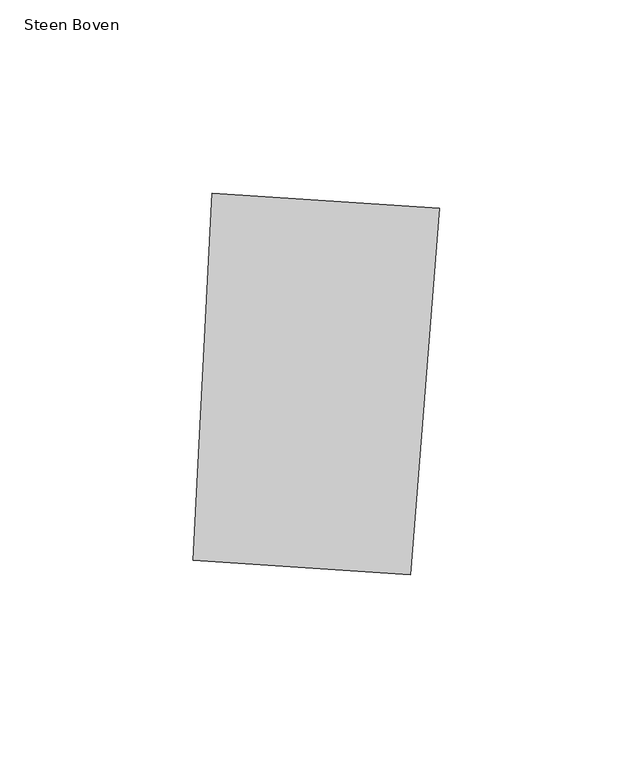
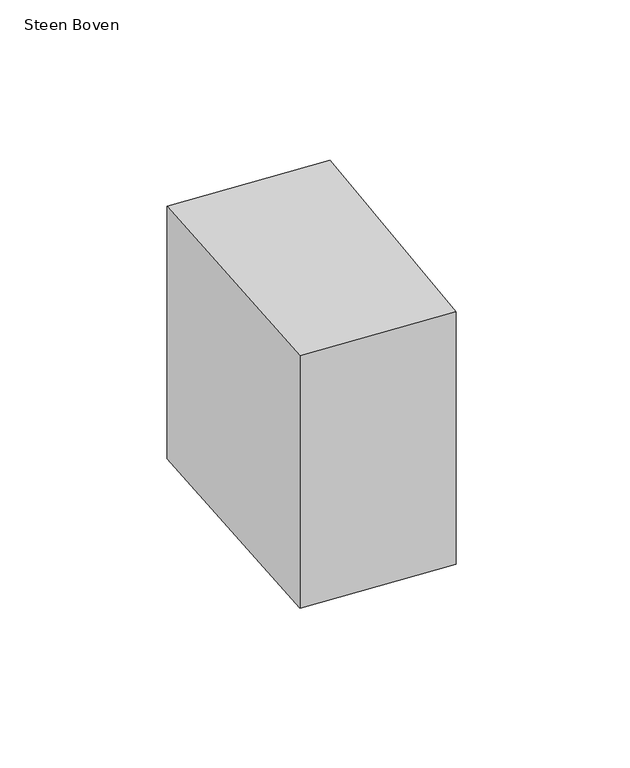
"""IFC4 building model written with IfcOpenShell, lengths in millimetres: proxy geometry, 00_GMA_steen_versie_4 : Steen Boven."""

import ifcopenshell
import ifcopenshell.guid

model = None  # the IFC model being written
_history = None  # IfcOwnerHistory: only IFC2X3 demands one
_inside = {}  # id of a spatial element -> (the spatial element, [elements in it])
_under = {}  # id of a project, library or spatial element -> (it, [spatial elements below it])
_declared = {}  # id of a project -> (the project, [libraries it declares])
_typed = {}  # id of a type object -> (the type object, [elements of that type])
_made_of = {}  # id of a material, layer set ... -> (it, [elements and type objects made of it])


def new_model(schema):
    """Start an empty IFC model of exactly this schema.

    Asked for "IFC4X3", IfcOpenShell would pick the latest addendum, in which some entities
    have other attributes; the version numbers below select the first issue.
    IFC2X3 requires an IfcOwnerHistory on every rooted entity: one is made here for all.
    """
    global model, _history
    if schema == "IFC4X3":
        model = ifcopenshell.file(schema_version=(4, 3, 0, 0))
    else:
        model = ifcopenshell.file(schema=schema)
    _inside.clear()
    _under.clear()
    _declared.clear()
    _typed.clear()
    _made_of.clear()
    _history = None
    if model.schema == "IFC2X3":
        org = make("IfcOrganization", Name="unknown")
        user = make(
            "IfcPersonAndOrganization",
            ThePerson=make("IfcPerson", FamilyName="unknown"),
            TheOrganization=org,
        )
        app = make(
            "IfcApplication",
            ApplicationDeveloper=org,
            Version="unknown",
            ApplicationFullName="unknown",
            ApplicationIdentifier="unknown",
        )
        _history = make(
            "IfcOwnerHistory",
            OwningUser=user,
            OwningApplication=app,
            ChangeAction="ADDED",
            CreationDate=0,
        )
    return model


def make(cls, **values):
    """One entity of the class cls with the attributes given. An attribute that is None is left unset."""
    return model.create_entity(
        cls, **{name: value for name, value in values.items() if value is not None}
    )


def rooted(cls, **values):
    """An entity with a GlobalId (a new one), such as an element, a storey or a relation."""
    return make(cls, GlobalId=ifcopenshell.guid.new(), OwnerHistory=_history, **values)


def si_unit(unit_type, name, prefix=None):
    """IfcSIUnit, for example si_unit("LENGTHUNIT", "METRE", prefix="MILLI")."""
    return make("IfcSIUnit", UnitType=unit_type, Prefix=prefix, Name=name)


def assignment(units):
    """IfcUnitAssignment: the units of a project."""
    return None if units is None else make("IfcUnitAssignment", Units=units)


def point(xyz):
    """IfcCartesianPoint."""
    return None if xyz is None else make("IfcCartesianPoint", Coordinates=xyz)


def direction(xyz):
    """IfcDirection."""
    return None if xyz is None else make("IfcDirection", DirectionRatios=xyz)


def frame(location, z_axis=None, x_axis=None):
    """IfcAxis2Placement3D, a coordinate frame: its origin and axes. An axis left out is left unset."""
    return make(
        "IfcAxis2Placement3D",
        Location=point(location),
        Axis=direction(z_axis),
        RefDirection=direction(x_axis),
    )


def origin():
    """The frame at (0, 0, 0) with its axes left unset."""
    return frame((0.0, 0.0, 0.0))


def origin_with_axes():
    """The frame at (0, 0, 0) with the z axis (0, 0, 1) and the x axis (1, 0, 0) written out."""
    return frame((0.0, 0.0, 0.0), z_axis=(0.0, 0.0, 1.0), x_axis=(1.0, 0.0, 0.0))


def place(relative_to, where):
    """IfcLocalPlacement: puts the frame where relative to a parent placement (None: the world)."""
    return make(
        "IfcLocalPlacement", PlacementRelTo=relative_to, RelativePlacement=where
    )


def context(
    kind, dimensions, precision=None, world=None, true_north=None, identifier=None
):
    """IfcGeometricRepresentationContext, for example the 3D "Model" context."""
    return make(
        "IfcGeometricRepresentationContext",
        ContextIdentifier=identifier,
        ContextType=kind,
        CoordinateSpaceDimension=dimensions,
        Precision=precision,
        WorldCoordinateSystem=world,
        TrueNorth=true_north,
    )


def project(units=None, contexts=None):
    """IfcProject with its units and contexts."""
    return rooted(
        "IfcProject",
        Name="project",
        RepresentationContexts=contexts,
        UnitsInContext=assignment(units),
    )


def spatial(cls, under=None, at=None, **own):
    """A site, building, storey or space (cls), placed at a placement, below another one or the project."""
    s = rooted(cls, ObjectPlacement=at, **own)
    if under is not None:
        _under.setdefault(under.id(), (under, []))[1].append(s)
    return s


def polyline(points):
    """IfcPolyline through the points."""
    return make("IfcPolyline", Points=[point(p) for p in points])


def outline(outer, holes=None, kind="AREA"):
    """IfcArbitraryClosedProfileDef: a profile drawn as a closed curve; with holes, ...WithVoids."""
    if holes is None:
        return make("IfcArbitraryClosedProfileDef", ProfileType=kind, OuterCurve=outer)
    return make(
        "IfcArbitraryProfileDefWithVoids",
        ProfileType=kind,
        OuterCurve=outer,
        InnerCurves=holes,
    )


def extrude(swept, where, along, depth):
    """IfcExtrudedAreaSolid: the profile swept, set in the frame where, extruded along a direction by depth."""
    return make(
        "IfcExtrudedAreaSolid",
        SweptArea=swept,
        Position=where,
        ExtrudedDirection=direction(along),
        Depth=depth,
    )


def shape(context_of_items, identifier, shape_type, items):
    """IfcShapeRepresentation: the items that make up one representation, for example the "Body"."""
    return make(
        "IfcShapeRepresentation",
        ContextOfItems=context_of_items,
        RepresentationIdentifier=identifier,
        RepresentationType=shape_type,
        Items=items,
    )


def source(mapping_origin, context_of_items, identifier, shape_type, items):
    """IfcRepresentationMap: a shape defined once, which mapped items show again and again."""
    return make(
        "IfcRepresentationMap",
        MappingOrigin=mapping_origin,
        MappedRepresentation=shape(context_of_items, identifier, shape_type, items),
    )


def transform(
    local_origin,
    x_axis=None,
    y_axis=None,
    z_axis=None,
    scale=None,
    scale2=None,
    scale3=None,
    uniform=True,
):
    """IfcCartesianTransformationOperator3D, or its non-uniform kind. x_axis, y_axis, z_axis: its Axis1, 2, 3."""
    if uniform:
        return make(
            "IfcCartesianTransformationOperator3D",
            Axis1=direction(x_axis),
            Axis2=direction(y_axis),
            LocalOrigin=point(local_origin),
            Scale=scale,
            Axis3=direction(z_axis),
        )
    return make(
        "IfcCartesianTransformationOperator3DnonUniform",
        Axis1=direction(x_axis),
        Axis2=direction(y_axis),
        LocalOrigin=point(local_origin),
        Scale=scale,
        Axis3=direction(z_axis),
        Scale2=scale2,
        Scale3=scale3,
    )


def mapped(mapping_source, mapping_target):
    """IfcMappedItem: shows the shape of a source again, moved by a transform."""
    return make(
        "IfcMappedItem", MappingSource=mapping_source, MappingTarget=mapping_target
    )


def made_of(thing, what):
    """Note that an element or type object is made of a material, layer set ...; save() writes the relation."""
    if what is not None:
        _made_of.setdefault(what.id(), (what, []))[1].append(thing)
    return thing


def element(
    cls,
    number,
    at=None,
    inside=None,
    cuts=None,
    type_object=None,
    material=None,
    context=None,
    identifier="Body",
    shape_type=None,
    held_by="IfcProductDefinitionShape",
    body=None,
    shapes=None,
    **own,
):
    """One element of the class cls, such as IfcWall. Its Tag is "e" and its number.

    at: its placement. inside: the storey or other place that contains it. cuts: it is an
    opening in that element (IfcRelVoidsElement). A single representation is given by context,
    identifier, shape_type and body (its items); several are given by shapes. held_by: the class
    of the entity that holds the representations. save() writes the other relations.
    """
    e = rooted(cls, Tag="e%d" % number, ObjectPlacement=at, **own)
    if body is not None:
        shapes = [shape(context, identifier, shape_type, body)]
    if shapes is not None:
        e.Representation = make(held_by, Representations=shapes)
    if inside is not None:
        _inside.setdefault(inside.id(), (inside, []))[1].append(e)
    if cuts is not None:
        rooted(
            "IfcRelVoidsElement", RelatingBuildingElement=cuts, RelatedOpeningElement=e
        )
    if type_object is not None:
        _typed.setdefault(type_object.id(), (type_object, []))[1].append(e)
    return made_of(e, material)


def aggregate(whole, parts):
    """IfcRelAggregates: a whole, such as a stair, and the parts it consists of."""
    return rooted("IfcRelAggregates", RelatingObject=whole, RelatedObjects=parts)


def save(model, path):
    """Write the relations noted so far, then the file.

    IfcRelAggregates (storeys below a building ...), IfcRelContainedInSpatialStructure (elements
    in a storey), IfcRelDefinesByType, IfcRelAssociatesMaterial and IfcRelDeclares: one each for
    every whole, place, type object, material and project.
    """
    for whole, parts in _under.values():
        aggregate(whole, parts)
    for where, things in _inside.values():
        rooted(
            "IfcRelContainedInSpatialStructure",
            RelatedElements=things,
            RelatingStructure=where,
        )
    for kind, things in _typed.values():
        rooted("IfcRelDefinesByType", RelatedObjects=things, RelatingType=kind)
    for what, things in _made_of.values():
        rooted("IfcRelAssociatesMaterial", RelatedObjects=things, RelatingMaterial=what)
    for by, libraries in _declared.values():
        rooted("IfcRelDeclares", RelatingContext=by, RelatedDefinitions=libraries)
    model.write(path)


def steen_boven_22b2381c(model_context):
    return source(origin(), model_context, "Body", "SweptSolid", [
        extrude(outline(polyline([(104.5278242, 118.7712704), (96.9962785, 24.0607473), (40.7725182, 27.7522095), (45.6889916, 122.6344294), (104.5278242, 118.7712704)])), origin_with_axes(), (0.0, 0.0, 1.0), 100.0),
    ])


if __name__ == "__main__":
    model = new_model("IFC4")
    model_context = context("Model", 3, world=origin())
    ifc_project = project(units=[si_unit("LENGTHUNIT", "METRE", prefix="MILLI")], contexts=[model_context])
    site = spatial("IfcSite", under=ifc_project)
    building = spatial("IfcBuilding", under=site)
    placement = place(None, origin())
    steen_boven_shape = steen_boven_22b2381c(model_context)
    element("IfcBuildingElementProxy", 1, Name="00_GMA_steen_versie_4 : Steen Boven", ObjectType="00_GMA_steen_versie_4 : Steen Boven", at=placement, inside=building, context=model_context, shape_type="MappedRepresentation", body=[
        mapped(steen_boven_shape, transform((0.0, 0.0, 0.0), x_axis=(1.0, 0.0, 0.0), y_axis=(0.0, 1.0, 0.0), z_axis=(0.0, 0.0, 1.0))),
    ])
    save(model, "model.ifc")

# Revit data of these elements
# Type "00_GMA_steen_versie_4 : Steen Boven"
#   StootVoegHalfBoven [instance default] = 5 mm
#   StootVoegHalf [instance default] = 5 mm
#   StootVoegBreedteOnder = 10 mm
#   StootVoegBreedteBoven = 10 mm
#   Steendikte = 100 mm
#   LintVoegOnderHalf = 5 mm
#   LintVoegOnder = 10 mm
#   LintVoegBovenHalf = 0 mm
#   LintVoegBoven = 0 mm
#   materiaal = none
#   MateriaalVoeg = none
#   Default Elevation = 0
